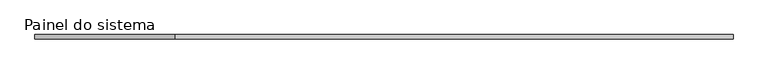
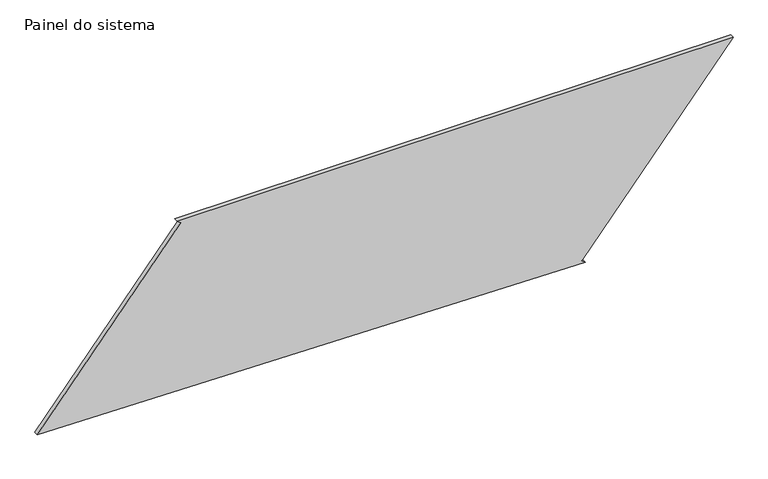
"""IFC4 building model written with IfcOpenShell, lengths in millimetres: plate geometry, Painel do sistema : Envidraçado."""

from ifc_helpers import new_model, si_unit, frame, origin, place, context, project, spatial, polyline, outline, extrude, source, transform, mapped, element, save


def painel_do_sistema_64eb0f9a(model_context):
    return source(origin(), model_context, "Body", "SweptSolid", [
        extrude(outline(polyline([(0.0, 1188.078409), (15.8992441, 1168.7855596), (1105.0633308, 2066.3660747), (1105.0633308, -1234.8945225), (1089.1640867, -1215.6016732), (56.8087527, -2066.3660747), (0.0, 1188.078409)])), frame((0.0, 24.5, 0.0), z_axis=(0.0, 1.0, 0.0), x_axis=(0.0, 0.0, 1.0)), (0.0, 0.0, 1.0), 25.0),
    ])


if __name__ == "__main__":
    model = new_model("IFC4")
    model_context = context("Model", 3, world=origin())
    ifc_project = project(units=[si_unit("LENGTHUNIT", "METRE", prefix="MILLI")], contexts=[model_context])
    site = spatial("IfcSite", under=ifc_project)
    building = spatial("IfcBuilding", under=site)
    placement = place(None, origin())
    painel_do_sistema_shape = painel_do_sistema_64eb0f9a(model_context)
    element("IfcPlate", 1, ObjectType="Painel do sistema : Envidraçado", at=placement, inside=building, context=model_context, shape_type="MappedRepresentation", body=[
        mapped(painel_do_sistema_shape, transform((0.0, 0.0, 0.0), x_axis=(1.0, 0.0, 0.0), y_axis=(0.0, 1.0, 0.0), z_axis=(0.0, 0.0, 1.0))),
    ])
    save(model, "model.ifc")

# Revit data of these elements
# Type "Painel do sistema : Envidraçado"
#   Construction Type Id = "GSP4R"
#   Analytic Construction = "Vidraça única Pilkington 1/8 pol"
#   Visual Light Transmittance = 0.9
#   Solar Heat Gain Coefficient = 0.86
#   Heat Transfer Coefficient (U) = 6.7069 W/(m²·K)
# Element 1 (IfcPlate, "Painel do sistema : Envidraçado")
#   Materials on its faces: "Vidro"
# Materials
#   "Vidro": class "Vidro", colour RGB 0 128 192, transparency 0.9, Description = "Vidro de sílica", Cost = 0
